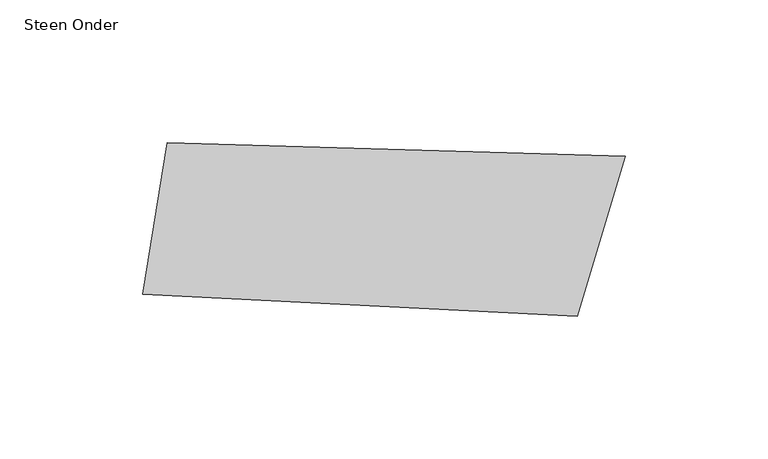
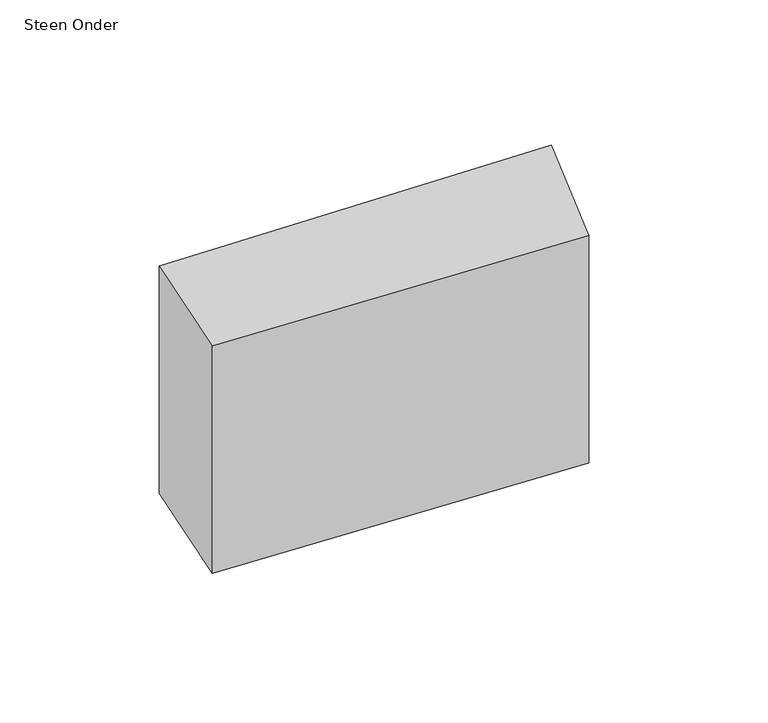
"""IFC4 building model written with IfcOpenShell, lengths in millimetres: proxy geometry, 00_GMA_steen_versie_4 : Steen Onder."""

from ifc_helpers import new_model, si_unit, frame, origin, place, context, project, spatial, polyline, outline, extrude, source, transform, mapped, element, save


def steen_onder_7475fe11(model_context):
    return source(origin(), model_context, "Body", "SweptSolid", [
        extrude(outline(polyline([(182.2822469, 61.4507991), (165.5052902, 5.4323842), (13.3217124, 13.0722395), (21.9311274, 66.1134233), (182.2822469, 61.4507991)])), frame((0.0, 0.0, -100.0), z_axis=(0.0, 0.0, 1.0), x_axis=(1.0, 0.0, 0.0)), (0.0, 0.0, 1.0), 100.0),
    ])


if __name__ == "__main__":
    model = new_model("IFC4")
    model_context = context("Model", 3, world=origin())
    ifc_project = project(units=[si_unit("LENGTHUNIT", "METRE", prefix="MILLI")], contexts=[model_context])
    site = spatial("IfcSite", under=ifc_project)
    building = spatial("IfcBuilding", under=site)
    placement = place(None, origin())
    steen_onder_shape = steen_onder_7475fe11(model_context)
    element("IfcBuildingElementProxy", 1, Name="00_GMA_steen_versie_4 : Steen Onder", ObjectType="00_GMA_steen_versie_4 : Steen Onder", at=placement, inside=building, context=model_context, shape_type="MappedRepresentation", body=[
        mapped(steen_onder_shape, transform((0.0, 0.0, 0.0), x_axis=(1.0, 0.0, 0.0), y_axis=(0.0, 1.0, 0.0), z_axis=(0.0, 0.0, 1.0))),
    ])
    save(model, "model.ifc")

# Revit data of these elements
# Type "00_GMA_steen_versie_4 : Steen Onder"
#   StootVoegHalfBoven [instance default] = 5 mm
#   StootVoegHalf [instance default] = 5 mm
#   StootVoegBreedteOnder = 10 mm
#   StootVoegBreedteBoven = 10 mm
#   Steendikte = 100 mm
#   LintVoegOnderHalf = 0 mm
#   LintVoegOnder = 0 mm
#   LintVoegBovenHalf = 5 mm
#   LintVoegBoven = 10 mm
#   materiaal = none
#   MateriaalVoeg = none
#   Default Elevation = 0
